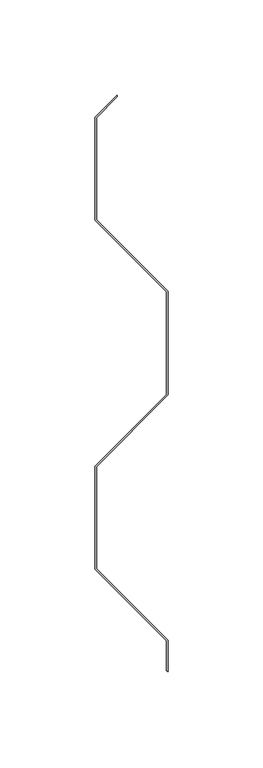
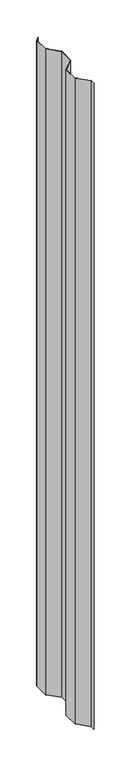
"""IFC4 building model written with IfcOpenShell, lengths in millimetres: proxy geometry, MBCI 7.2-V Panel33 : MBCI 7.2-V Panel-1."""

import ifcopenshell
import ifcopenshell.guid

model = None  # the IFC model being written
_history = None  # IfcOwnerHistory: only IFC2X3 demands one
_inside = {}  # id of a spatial element -> (the spatial element, [elements in it])
_under = {}  # id of a project, library or spatial element -> (it, [spatial elements below it])
_declared = {}  # id of a project -> (the project, [libraries it declares])
_typed = {}  # id of a type object -> (the type object, [elements of that type])
_made_of = {}  # id of a material, layer set ... -> (it, [elements and type objects made of it])


def new_model(schema):
    """Start an empty IFC model of exactly this schema.

    Asked for "IFC4X3", IfcOpenShell would pick the latest addendum, in which some entities
    have other attributes; the version numbers below select the first issue.
    IFC2X3 requires an IfcOwnerHistory on every rooted entity: one is made here for all.
    """
    global model, _history
    if schema == "IFC4X3":
        model = ifcopenshell.file(schema_version=(4, 3, 0, 0))
    else:
        model = ifcopenshell.file(schema=schema)
    _inside.clear()
    _under.clear()
    _declared.clear()
    _typed.clear()
    _made_of.clear()
    _history = None
    if model.schema == "IFC2X3":
        org = make("IfcOrganization", Name="unknown")
        user = make(
            "IfcPersonAndOrganization",
            ThePerson=make("IfcPerson", FamilyName="unknown"),
            TheOrganization=org,
        )
        app = make(
            "IfcApplication",
            ApplicationDeveloper=org,
            Version="unknown",
            ApplicationFullName="unknown",
            ApplicationIdentifier="unknown",
        )
        _history = make(
            "IfcOwnerHistory",
            OwningUser=user,
            OwningApplication=app,
            ChangeAction="ADDED",
            CreationDate=0,
        )
    return model


def make(cls, **values):
    """One entity of the class cls with the attributes given. An attribute that is None is left unset."""
    return model.create_entity(
        cls, **{name: value for name, value in values.items() if value is not None}
    )


def rooted(cls, **values):
    """An entity with a GlobalId (a new one), such as an element, a storey or a relation."""
    return make(cls, GlobalId=ifcopenshell.guid.new(), OwnerHistory=_history, **values)


def si_unit(unit_type, name, prefix=None):
    """IfcSIUnit, for example si_unit("LENGTHUNIT", "METRE", prefix="MILLI")."""
    return make("IfcSIUnit", UnitType=unit_type, Prefix=prefix, Name=name)


def assignment(units):
    """IfcUnitAssignment: the units of a project."""
    return None if units is None else make("IfcUnitAssignment", Units=units)


def point(xyz):
    """IfcCartesianPoint."""
    return None if xyz is None else make("IfcCartesianPoint", Coordinates=xyz)


def direction(xyz):
    """IfcDirection."""
    return None if xyz is None else make("IfcDirection", DirectionRatios=xyz)


def frame(location, z_axis=None, x_axis=None):
    """IfcAxis2Placement3D, a coordinate frame: its origin and axes. An axis left out is left unset."""
    return make(
        "IfcAxis2Placement3D",
        Location=point(location),
        Axis=direction(z_axis),
        RefDirection=direction(x_axis),
    )


def origin():
    """The frame at (0, 0, 0) with its axes left unset."""
    return frame((0.0, 0.0, 0.0))


def origin_with_axes():
    """The frame at (0, 0, 0) with the z axis (0, 0, 1) and the x axis (1, 0, 0) written out."""
    return frame((0.0, 0.0, 0.0), z_axis=(0.0, 0.0, 1.0), x_axis=(1.0, 0.0, 0.0))


def place(relative_to, where):
    """IfcLocalPlacement: puts the frame where relative to a parent placement (None: the world)."""
    return make(
        "IfcLocalPlacement", PlacementRelTo=relative_to, RelativePlacement=where
    )


def context(
    kind, dimensions, precision=None, world=None, true_north=None, identifier=None
):
    """IfcGeometricRepresentationContext, for example the 3D "Model" context."""
    return make(
        "IfcGeometricRepresentationContext",
        ContextIdentifier=identifier,
        ContextType=kind,
        CoordinateSpaceDimension=dimensions,
        Precision=precision,
        WorldCoordinateSystem=world,
        TrueNorth=true_north,
    )


def project(units=None, contexts=None):
    """IfcProject with its units and contexts."""
    return rooted(
        "IfcProject",
        Name="project",
        RepresentationContexts=contexts,
        UnitsInContext=assignment(units),
    )


def spatial(cls, under=None, at=None, **own):
    """A site, building, storey or space (cls), placed at a placement, below another one or the project."""
    s = rooted(cls, ObjectPlacement=at, **own)
    if under is not None:
        _under.setdefault(under.id(), (under, []))[1].append(s)
    return s


def polyline(points):
    """IfcPolyline through the points."""
    return make("IfcPolyline", Points=[point(p) for p in points])


def outline(outer, holes=None, kind="AREA"):
    """IfcArbitraryClosedProfileDef: a profile drawn as a closed curve; with holes, ...WithVoids."""
    if holes is None:
        return make("IfcArbitraryClosedProfileDef", ProfileType=kind, OuterCurve=outer)
    return make(
        "IfcArbitraryProfileDefWithVoids",
        ProfileType=kind,
        OuterCurve=outer,
        InnerCurves=holes,
    )


def extrude(swept, where, along, depth):
    """IfcExtrudedAreaSolid: the profile swept, set in the frame where, extruded along a direction by depth."""
    return make(
        "IfcExtrudedAreaSolid",
        SweptArea=swept,
        Position=where,
        ExtrudedDirection=direction(along),
        Depth=depth,
    )


def shape(context_of_items, identifier, shape_type, items):
    """IfcShapeRepresentation: the items that make up one representation, for example the "Body"."""
    return make(
        "IfcShapeRepresentation",
        ContextOfItems=context_of_items,
        RepresentationIdentifier=identifier,
        RepresentationType=shape_type,
        Items=items,
    )


def source(mapping_origin, context_of_items, identifier, shape_type, items):
    """IfcRepresentationMap: a shape defined once, which mapped items show again and again."""
    return make(
        "IfcRepresentationMap",
        MappingOrigin=mapping_origin,
        MappedRepresentation=shape(context_of_items, identifier, shape_type, items),
    )


def transform(
    local_origin,
    x_axis=None,
    y_axis=None,
    z_axis=None,
    scale=None,
    scale2=None,
    scale3=None,
    uniform=True,
):
    """IfcCartesianTransformationOperator3D, or its non-uniform kind. x_axis, y_axis, z_axis: its Axis1, 2, 3."""
    if uniform:
        return make(
            "IfcCartesianTransformationOperator3D",
            Axis1=direction(x_axis),
            Axis2=direction(y_axis),
            LocalOrigin=point(local_origin),
            Scale=scale,
            Axis3=direction(z_axis),
        )
    return make(
        "IfcCartesianTransformationOperator3DnonUniform",
        Axis1=direction(x_axis),
        Axis2=direction(y_axis),
        LocalOrigin=point(local_origin),
        Scale=scale,
        Axis3=direction(z_axis),
        Scale2=scale2,
        Scale3=scale3,
    )


def mapped(mapping_source, mapping_target):
    """IfcMappedItem: shows the shape of a source again, moved by a transform."""
    return make(
        "IfcMappedItem", MappingSource=mapping_source, MappingTarget=mapping_target
    )


def made_of(thing, what):
    """Note that an element or type object is made of a material, layer set ...; save() writes the relation."""
    if what is not None:
        _made_of.setdefault(what.id(), (what, []))[1].append(thing)
    return thing


def element(
    cls,
    number,
    at=None,
    inside=None,
    cuts=None,
    type_object=None,
    material=None,
    context=None,
    identifier="Body",
    shape_type=None,
    held_by="IfcProductDefinitionShape",
    body=None,
    shapes=None,
    **own,
):
    """One element of the class cls, such as IfcWall. Its Tag is "e" and its number.

    at: its placement. inside: the storey or other place that contains it. cuts: it is an
    opening in that element (IfcRelVoidsElement). A single representation is given by context,
    identifier, shape_type and body (its items); several are given by shapes. held_by: the class
    of the entity that holds the representations. save() writes the other relations.
    """
    e = rooted(cls, Tag="e%d" % number, ObjectPlacement=at, **own)
    if body is not None:
        shapes = [shape(context, identifier, shape_type, body)]
    if shapes is not None:
        e.Representation = make(held_by, Representations=shapes)
    if inside is not None:
        _inside.setdefault(inside.id(), (inside, []))[1].append(e)
    if cuts is not None:
        rooted(
            "IfcRelVoidsElement", RelatingBuildingElement=cuts, RelatedOpeningElement=e
        )
    if type_object is not None:
        _typed.setdefault(type_object.id(), (type_object, []))[1].append(e)
    return made_of(e, material)


def aggregate(whole, parts):
    """IfcRelAggregates: a whole, such as a stair, and the parts it consists of."""
    return rooted("IfcRelAggregates", RelatingObject=whole, RelatedObjects=parts)


def save(model, path):
    """Write the relations noted so far, then the file.

    IfcRelAggregates (storeys below a building ...), IfcRelContainedInSpatialStructure (elements
    in a storey), IfcRelDefinesByType, IfcRelAssociatesMaterial and IfcRelDeclares: one each for
    every whole, place, type object, material and project.
    """
    for whole, parts in _under.values():
        aggregate(whole, parts)
    for where, things in _inside.values():
        rooted(
            "IfcRelContainedInSpatialStructure",
            RelatedElements=things,
            RelatingStructure=where,
        )
    for kind, things in _typed.values():
        rooted("IfcRelDefinesByType", RelatedObjects=things, RelatingType=kind)
    for what, things in _made_of.values():
        rooted("IfcRelAssociatesMaterial", RelatedObjects=things, RelatingMaterial=what)
    for by, libraries in _declared.values():
        rooted("IfcRelDeclares", RelatingContext=by, RelatedDefinitions=libraries)
    model.write(path)


def generic_models_5c371aaf(model_context):
    return source(origin(), model_context, "Body", "SweptSolid", [
        extrude(outline(polyline([(590353.5827614, -536183.1919067), (590353.5827614, -536129.0801976), (590364.9833956, -536117.6795634), (590365.0253204, -536118.4795376), (590354.1780739, -536129.3267841), (590354.1780739, -536182.9453202), (590391.6684739, -536220.4357202), (590391.6684739, -536274.7163841), (590354.1780739, -536312.2067841), (590354.1780739, -536365.8253202), (590391.6684739, -536403.3157202), (590391.6684739, -536419.8041735), (590391.0731614, -536419.2866763), (590391.0731614, -536403.5623067), (590353.5827614, -536366.0719067), (590353.5827614, -536311.9601976), (590391.0731614, -536274.4697976), (590391.0731614, -536220.6823067), (590353.5827614, -536183.1919067)])), origin_with_axes(), (0.0, 0.0, 1.0), 2438.4),
    ])


if __name__ == "__main__":
    model = new_model("IFC4")
    model_context = context("Model", 3, world=origin())
    ifc_project = project(units=[si_unit("LENGTHUNIT", "METRE", prefix="MILLI")], contexts=[model_context])
    site = spatial("IfcSite", under=ifc_project)
    building = spatial("IfcBuilding", under=site)
    placement = place(None, origin())
    generic_models_shape = generic_models_5c371aaf(model_context)
    element("IfcBuildingElementProxy", 1, Name="MBCI 7.2-V Panel33 : MBCI 7.2-V Panel-1", ObjectType="MBCI 7.2-V Panel33 : MBCI 7.2-V Panel-1", at=placement, inside=building, context=model_context, shape_type="MappedRepresentation", body=[
        mapped(generic_models_shape, transform((0.0, 0.0, 0.0), x_axis=(1.0, 0.0, 0.0), y_axis=(0.0, 1.0, 0.0), z_axis=(0.0, 0.0, 1.0))),
    ])
    save(model, "model.ifc")

# Revit data of these elements
# Element 1 (IfcBuildingElementProxy, "MBCI 7.2-V Panel33 : MBCI 7.2-V Panel-1")
#   Materials on its faces: "MTL PANEL"
# Materials
#   "MTL PANEL": class "Generic", colour RGB 239 242 240, transparency 0, Cost = 0
